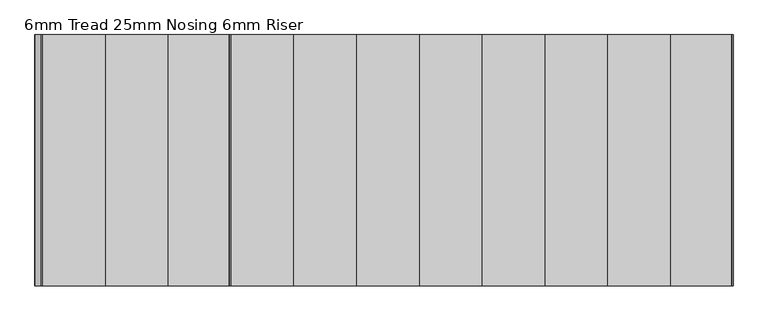
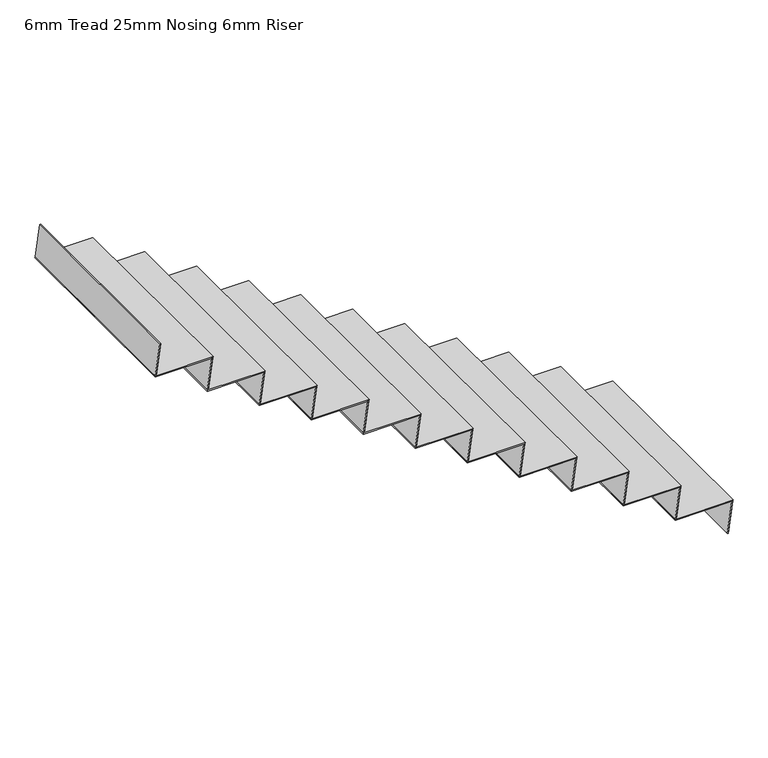
"""IFC4 building model written with IfcOpenShell, lengths in millimetres: stair flight geometry, 6mm Tread 25mm Nosing 6mm Riser."""

from ifc_helpers import new_model, si_unit, origin, place, context, project, spatial, faceted_brep, source, transform, mapped, element, save


def stair_flight_6mm_tread_25mm_nosing_6mm_riser_fe0d3516(model_context):
    return source(origin(), model_context, "Body", "Brep", [
        faceted_brep([(-13631.0599092, 11395.4345331, 20176.4705882), (-13631.9099092, 11395.4345331, 20170.4705882), (-13631.9099092, 10295.4345331, 20170.4705882), (-13631.0599092, 10295.4345331, 20176.4705882), (-13325.0, 10295.4345331, 20176.4705882), (-13325.0, 11395.4345331, 20176.4705882), (-13325.85, 11395.4345331, 20170.4705882), (-13325.85, 10295.4345331, 20170.4705882)], [[[0, 1, 2, 3]], [[3, 4, 5, 0]], [[2, 1, 6, 7]], [[4, 3, 2, 7]], [[0, 5, 6, 1]], [[5, 4, 7, 6]]]),
        faceted_brep([(-13325.85, 11395.4345331, 20170.4705882), (-13350.0, 11395.4345331, 20000.0), (-13356.0599092, 11395.4345331, 20000.0), (-13331.9099092, 11395.4345331, 20170.4705882), (-13325.85, 10295.4345331, 20170.4705882), (-13331.9099092, 10295.4345331, 20170.4705882), (-13356.0599092, 10295.4345331, 20000.0), (-13350.0, 10295.4345331, 20000.0)], [[[0, 1, 2, 3]], [[4, 5, 6, 7]], [[1, 0, 4, 7]], [[2, 1, 7, 6]], [[3, 2, 6, 5]], [[0, 3, 5, 4]]]),
        faceted_brep([(-13600.85, 11395.4345331, 20346.9411765), (-13625.0, 11395.4345331, 20176.4705882), (-13631.0599092, 11395.4345331, 20176.4705882), (-13606.9099092, 11395.4345331, 20346.9411765), (-13600.85, 10295.4345331, 20346.9411765), (-13606.9099092, 10295.4345331, 20346.9411765), (-13631.0599092, 10295.4345331, 20176.4705882), (-13625.0, 10295.4345331, 20176.4705882)], [[[0, 1, 2, 3]], [[4, 5, 6, 7]], [[1, 0, 4, 7]], [[2, 1, 7, 6]], [[3, 2, 6, 5]], [[0, 3, 5, 4]]]),
        faceted_brep([(-13906.0599092, 10295.4345331, 20352.9411765), (-13600.0, 10295.4345331, 20352.9411765), (-13600.0, 11395.4345331, 20352.9411765), (-13906.0599092, 11395.4345331, 20352.9411765), (-13906.9099092, 10295.4345331, 20346.9411765), (-13906.9099092, 11395.4345331, 20346.9411765), (-13600.85, 11395.4345331, 20346.9411765), (-13600.85, 10295.4345331, 20346.9411765)], [[[0, 1, 2, 3]], [[4, 5, 6, 7]], [[1, 0, 4, 7]], [[3, 2, 6, 5]], [[3, 5, 4, 0]], [[2, 1, 7, 6]]]),
        faceted_brep([(-13875.85, 11395.4345331, 20523.4117647), (-13900.0, 11395.4345331, 20352.9411765), (-13906.0599092, 11395.4345331, 20352.9411765), (-13881.9099092, 11395.4345331, 20523.4117647), (-13875.85, 10295.4345331, 20523.4117647), (-13881.9099092, 10295.4345331, 20523.4117647), (-13906.0599092, 10295.4345331, 20352.9411765), (-13900.0, 10295.4345331, 20352.9411765)], [[[0, 1, 2, 3]], [[4, 5, 6, 7]], [[1, 0, 4, 7]], [[2, 1, 7, 6]], [[3, 2, 6, 5]], [[0, 3, 5, 4]]]),
        faceted_brep([(-14181.0599092, 10295.4345331, 20529.4117647), (-13875.0, 10295.4345331, 20529.4117647), (-13875.0, 11395.4345331, 20529.4117647), (-14181.0599092, 11395.4345331, 20529.4117647), (-14181.9099092, 10295.4345331, 20523.4117647), (-14181.9099092, 11395.4345331, 20523.4117647), (-13875.85, 11395.4345331, 20523.4117647), (-13875.85, 10295.4345331, 20523.4117647)], [[[0, 1, 2, 3]], [[4, 5, 6, 7]], [[1, 0, 4, 7]], [[3, 2, 6, 5]], [[3, 5, 4, 0]], [[2, 1, 7, 6]]]),
        faceted_brep([(-14150.85, 11395.4345331, 20699.8823529), (-14175.0, 11395.4345331, 20529.4117647), (-14181.0599092, 11395.4345331, 20529.4117647), (-14156.9099092, 11395.4345331, 20699.8823529), (-14150.85, 10295.4345331, 20699.8823529), (-14156.9099092, 10295.4345331, 20699.8823529), (-14181.0599092, 10295.4345331, 20529.4117647), (-14175.0, 10295.4345331, 20529.4117647)], [[[0, 1, 2, 3]], [[4, 5, 6, 7]], [[1, 0, 4, 7]], [[2, 1, 7, 6]], [[3, 2, 6, 5]], [[0, 3, 5, 4]]]),
        faceted_brep([(-14456.0599092, 10295.4345331, 20705.8823529), (-14150.0, 10295.4345331, 20705.8823529), (-14150.0, 11395.4345331, 20705.8823529), (-14456.0599092, 11395.4345331, 20705.8823529), (-14456.9099092, 10295.4345331, 20699.8823529), (-14456.9099092, 11395.4345331, 20699.8823529), (-14150.85, 11395.4345331, 20699.8823529), (-14150.85, 10295.4345331, 20699.8823529)], [[[0, 1, 2, 3]], [[4, 5, 6, 7]], [[1, 0, 4, 7]], [[3, 2, 6, 5]], [[3, 5, 4, 0]], [[2, 1, 7, 6]]]),
        faceted_brep([(-14425.85, 11395.4345331, 20876.3529412), (-14450.0, 11395.4345331, 20705.8823529), (-14456.0599092, 11395.4345331, 20705.8823529), (-14431.9099092, 11395.4345331, 20876.3529412), (-14425.85, 10295.4345331, 20876.3529412), (-14431.9099092, 10295.4345331, 20876.3529412), (-14456.0599092, 10295.4345331, 20705.8823529), (-14450.0, 10295.4345331, 20705.8823529)], [[[0, 1, 2, 3]], [[4, 5, 6, 7]], [[1, 0, 4, 7]], [[2, 1, 7, 6]], [[3, 2, 6, 5]], [[0, 3, 5, 4]]]),
        faceted_brep([(-14731.0599092, 10295.4345331, 20882.3529412), (-14425.0, 10295.4345331, 20882.3529412), (-14425.0, 11395.4345331, 20882.3529412), (-14731.0599092, 11395.4345331, 20882.3529412), (-14731.9099092, 10295.4345331, 20876.3529412), (-14731.9099092, 11395.4345331, 20876.3529412), (-14425.85, 11395.4345331, 20876.3529412), (-14425.85, 10295.4345331, 20876.3529412)], [[[0, 1, 2, 3]], [[4, 5, 6, 7]], [[1, 0, 4, 7]], [[3, 2, 6, 5]], [[3, 5, 4, 0]], [[2, 1, 7, 6]]]),
        faceted_brep([(-14700.85, 11395.4345331, 21052.8235294), (-14725.0, 11395.4345331, 20882.3529412), (-14731.0599092, 11395.4345331, 20882.3529412), (-14706.9099092, 11395.4345331, 21052.8235294), (-14700.85, 10295.4345331, 21052.8235294), (-14706.9099092, 10295.4345331, 21052.8235294), (-14731.0599092, 10295.4345331, 20882.3529412), (-14725.0, 10295.4345331, 20882.3529412)], [[[0, 1, 2, 3]], [[4, 5, 6, 7]], [[1, 0, 4, 7]], [[2, 1, 7, 6]], [[3, 2, 6, 5]], [[0, 3, 5, 4]]]),
        faceted_brep([(-15006.0599092, 10295.4345331, 21058.8235294), (-14700.0, 10295.4345331, 21058.8235294), (-14700.0, 11395.4345331, 21058.8235294), (-15006.0599092, 11395.4345331, 21058.8235294), (-15006.9099092, 10295.4345331, 21052.8235294), (-15006.9099092, 11395.4345331, 21052.8235294), (-14700.85, 11395.4345331, 21052.8235294), (-14700.85, 10295.4345331, 21052.8235294)], [[[0, 1, 2, 3]], [[4, 5, 6, 7]], [[1, 0, 4, 7]], [[3, 2, 6, 5]], [[3, 5, 4, 0]], [[2, 1, 7, 6]]]),
        faceted_brep([(-14975.85, 11395.4345331, 21229.2941176), (-15000.0, 11395.4345331, 21058.8235294), (-15006.0599092, 11395.4345331, 21058.8235294), (-14981.9099092, 11395.4345331, 21229.2941176), (-14975.85, 10295.4345331, 21229.2941176), (-14981.9099092, 10295.4345331, 21229.2941176), (-15006.0599092, 10295.4345331, 21058.8235294), (-15000.0, 10295.4345331, 21058.8235294)], [[[0, 1, 2, 3]], [[4, 5, 6, 7]], [[1, 0, 4, 7]], [[2, 1, 7, 6]], [[3, 2, 6, 5]], [[0, 3, 5, 4]]]),
        faceted_brep([(-15281.0599092, 10295.4345331, 21235.2941176), (-14975.0, 10295.4345331, 21235.2941176), (-14975.0, 11395.4345331, 21235.2941176), (-15281.0599092, 11395.4345331, 21235.2941176), (-15281.9099092, 10295.4345331, 21229.2941176), (-15281.9099092, 11395.4345331, 21229.2941176), (-14975.85, 11395.4345331, 21229.2941176), (-14975.85, 10295.4345331, 21229.2941176)], [[[0, 1, 2, 3]], [[4, 5, 6, 7]], [[1, 0, 4, 7]], [[3, 2, 6, 5]], [[3, 5, 4, 0]], [[2, 1, 7, 6]]]),
        faceted_brep([(-15250.85, 11395.4345331, 21405.7647059), (-15275.0, 11395.4345331, 21235.2941176), (-15281.0599092, 11395.4345331, 21235.2941176), (-15256.9099092, 11395.4345331, 21405.7647059), (-15250.85, 10295.4345331, 21405.7647059), (-15256.9099092, 10295.4345331, 21405.7647059), (-15281.0599092, 10295.4345331, 21235.2941176), (-15275.0, 10295.4345331, 21235.2941176)], [[[0, 1, 2, 3]], [[4, 5, 6, 7]], [[1, 0, 4, 7]], [[2, 1, 7, 6]], [[3, 2, 6, 5]], [[0, 3, 5, 4]]]),
        faceted_brep([(-15556.0599092, 10295.4345331, 21411.7647059), (-15250.0, 10295.4345331, 21411.7647059), (-15250.0, 11395.4345331, 21411.7647059), (-15556.0599092, 11395.4345331, 21411.7647059), (-15556.9099092, 10295.4345331, 21405.7647059), (-15556.9099092, 11395.4345331, 21405.7647059), (-15250.85, 11395.4345331, 21405.7647059), (-15250.85, 10295.4345331, 21405.7647059)], [[[0, 1, 2, 3]], [[4, 5, 6, 7]], [[1, 0, 4, 7]], [[3, 2, 6, 5]], [[3, 5, 4, 0]], [[2, 1, 7, 6]]]),
        faceted_brep([(-15525.85, 11395.4345331, 21582.2352941), (-15550.0, 11395.4345331, 21411.7647059), (-15556.0599092, 11395.4345331, 21411.7647059), (-15531.9099092, 11395.4345331, 21582.2352941), (-15525.85, 10295.4345331, 21582.2352941), (-15531.9099092, 10295.4345331, 21582.2352941), (-15556.0599092, 10295.4345331, 21411.7647059), (-15550.0, 10295.4345331, 21411.7647059)], [[[0, 1, 2, 3]], [[4, 5, 6, 7]], [[1, 0, 4, 7]], [[2, 1, 7, 6]], [[3, 2, 6, 5]], [[0, 3, 5, 4]]]),
        faceted_brep([(-15831.0599092, 10295.4345331, 21588.2352941), (-15525.0, 10295.4345331, 21588.2352941), (-15525.0, 11395.4345331, 21588.2352941), (-15831.0599092, 11395.4345331, 21588.2352941), (-15831.9099092, 10295.4345331, 21582.2352941), (-15831.9099092, 11395.4345331, 21582.2352941), (-15525.85, 11395.4345331, 21582.2352941), (-15525.85, 10295.4345331, 21582.2352941)], [[[0, 1, 2, 3]], [[4, 5, 6, 7]], [[1, 0, 4, 7]], [[3, 2, 6, 5]], [[3, 5, 4, 0]], [[2, 1, 7, 6]]]),
        faceted_brep([(-15800.85, 11395.4345331, 21758.7058824), (-15825.0, 11395.4345331, 21588.2352941), (-15831.0599092, 11395.4345331, 21588.2352941), (-15806.9099092, 11395.4345331, 21758.7058824), (-15800.85, 10295.4345331, 21758.7058824), (-15806.9099092, 10295.4345331, 21758.7058824), (-15831.0599092, 10295.4345331, 21588.2352941), (-15825.0, 10295.4345331, 21588.2352941)], [[[0, 1, 2, 3]], [[4, 5, 6, 7]], [[1, 0, 4, 7]], [[2, 1, 7, 6]], [[3, 2, 6, 5]], [[0, 3, 5, 4]]]),
        faceted_brep([(-16106.0599092, 10295.4345331, 21764.7058824), (-15800.0, 10295.4345331, 21764.7058824), (-15800.0, 11395.4345331, 21764.7058824), (-16106.0599092, 11395.4345331, 21764.7058824), (-16106.9099092, 10295.4345331, 21758.7058824), (-16106.9099092, 11395.4345331, 21758.7058824), (-15800.85, 11395.4345331, 21758.7058824), (-15800.85, 10295.4345331, 21758.7058824)], [[[0, 1, 2, 3]], [[4, 5, 6, 7]], [[1, 0, 4, 7]], [[3, 2, 6, 5]], [[3, 5, 4, 0]], [[2, 1, 7, 6]]]),
        faceted_brep([(-16350.85, 11395.4345331, 22111.6470588), (-16375.0, 11395.4345331, 21941.1764706), (-16381.0599092, 11395.4345331, 21941.1764706), (-16356.9099092, 11395.4345331, 22111.6470588), (-16350.85, 10295.4345331, 22111.6470588), (-16356.9099092, 10295.4345331, 22111.6470588), (-16381.0599092, 10295.4345331, 21941.1764706), (-16375.0, 10295.4345331, 21941.1764706)], [[[0, 1, 2, 3]], [[4, 5, 6, 7]], [[1, 0, 4, 7]], [[2, 1, 7, 6]], [[3, 2, 6, 5]], [[0, 3, 5, 4]]]),
        faceted_brep([(-16075.85, 11395.4345331, 21935.1764706), (-16100.0, 11395.4345331, 21764.7058824), (-16106.0599092, 11395.4345331, 21764.7058824), (-16081.9099092, 11395.4345331, 21935.1764706), (-16075.85, 10295.4345331, 21935.1764706), (-16081.9099092, 10295.4345331, 21935.1764706), (-16106.0599092, 10295.4345331, 21764.7058824), (-16100.0, 10295.4345331, 21764.7058824)], [[[0, 1, 2, 3]], [[4, 5, 6, 7]], [[1, 0, 4, 7]], [[2, 1, 7, 6]], [[3, 2, 6, 5]], [[0, 3, 5, 4]]]),
        faceted_brep([(-16381.0599092, 10295.4345331, 21941.1764706), (-16350.0, 10295.4345331, 21941.1764706), (-16075.0, 10295.4345331, 21941.1764706), (-16075.0, 11395.4345331, 21941.1764706), (-16381.0599092, 11395.4345331, 21941.1764706), (-16381.9099092, 10295.4345331, 21935.1764706), (-16381.9099092, 11395.4345331, 21935.1764706), (-16075.85, 11395.4345331, 21935.1764706), (-16075.85, 10295.4345331, 21935.1764706), (-16350.0, 10295.4345331, 21935.1764706)], [[[0, 1, 2, 3, 4]], [[5, 6, 7, 8, 9]], [[1, 0, 5, 9]], [[2, 1, 9, 8]], [[4, 3, 7, 6]], [[4, 6, 5, 0]], [[3, 2, 8, 7]]]),
    ])


if __name__ == "__main__":
    model = new_model("IFC4")
    model_context = context("Model", 3, world=origin())
    ifc_project = project(units=[si_unit("LENGTHUNIT", "METRE", prefix="MILLI")], contexts=[model_context])
    site = spatial("IfcSite", under=ifc_project)
    building = spatial("IfcBuilding", under=site)
    placement = place(None, origin())
    stair_flight_6mm_tread_25mm_nosing_6mm_riser_shape = stair_flight_6mm_tread_25mm_nosing_6mm_riser_fe0d3516(model_context)
    element("IfcStairFlight", 1, ObjectType="6mm Tread 25mm Nosing 6mm Riser", at=placement, inside=building, context=model_context, shape_type="MappedRepresentation", body=[
        mapped(stair_flight_6mm_tread_25mm_nosing_6mm_riser_shape, transform((0.0, 0.0, 0.0), x_axis=(1.0, 0.0, 0.0), y_axis=(0.0, 1.0, 0.0), z_axis=(0.0, 0.0, 1.0))),
    ])
    save(model, "model.ifc")

# Revit data of these elements
# Element 1 (IfcStairFlight, "6mm Tread 25mm Nosing 6mm Riser")
#   Materials on its faces: "Steel, Paint Finish, Dark Gray"
# Materials
#   "Steel, Paint Finish, Dark Gray": class "Metal", colour RGB 89 89 89, transparency 0, Description = "Steel, paint finish, dark gray, glossy", Cost = 0
